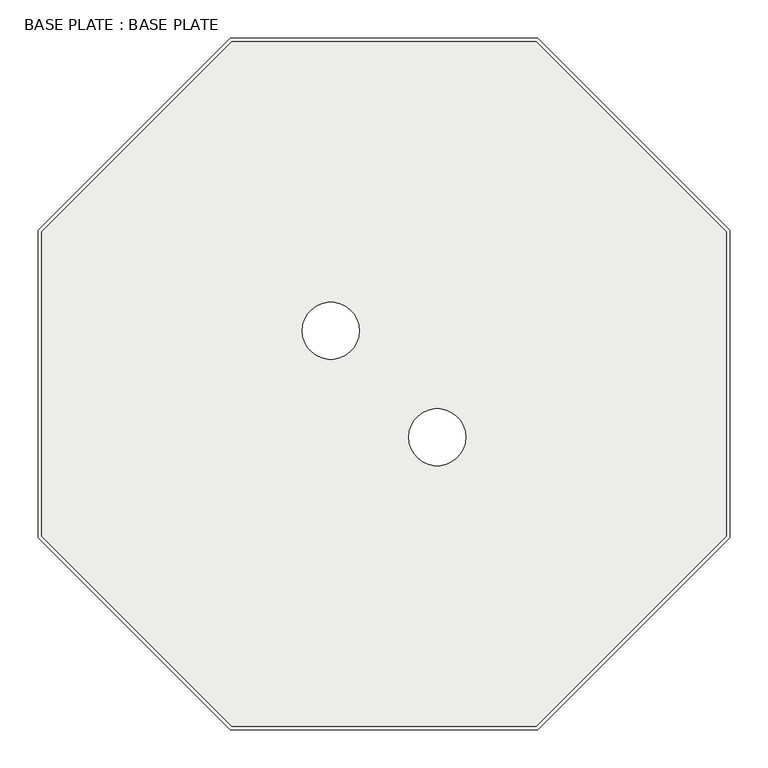
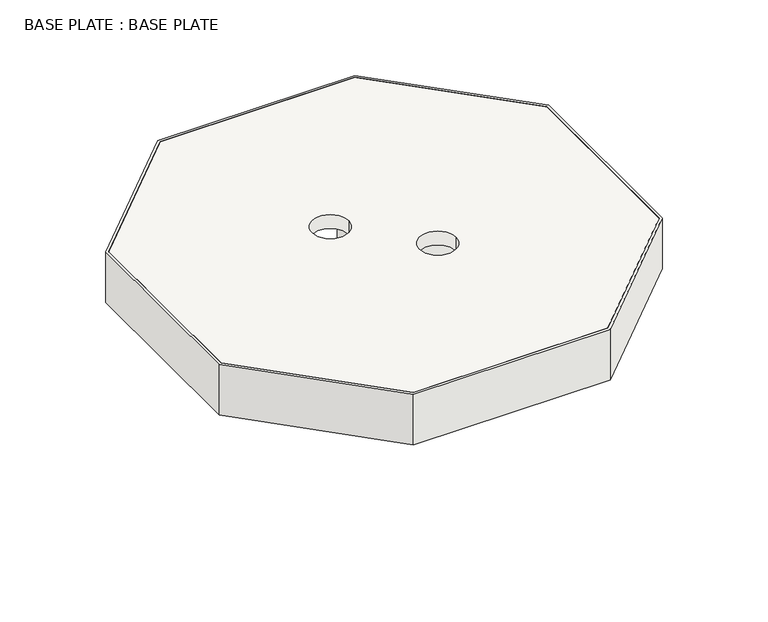
"""IFC4 building model written with IfcOpenShell, lengths in millimetres: slab geometry, BASE PLATE : BASE PLATE."""

from ifc_helpers import new_model, si_unit, point, frame, frame_2d, origin, place, context, project, spatial, polyline, circle_curve, trimmed, segment, composite_curve, outline, extrude, source, transform, mapped, element, save


def base_plate_base_plate_fc0de6f1(model_context):
    return source(origin(), model_context, "Body", "SweptSolid", [
        extrude(outline(polyline([(455.0, 19297.4497911), (202.0710678, 19044.5208589), (-202.0710678, 19044.5208589), (-455.0, 19297.4497911), (-455.0, 19701.5919267), (-202.0710678, 19954.5208589), (202.0710678, 19954.5208589), (455.0, 19701.5919267), (455.0, 19297.4497911)]), holes=[polyline([(-450.0, 19299.5208589), (-200.0, 19049.5208589), (200.0, 19049.5208589), (450.0, 19299.5208589), (450.0, 19699.5208589), (200.0, 19949.5208589), (-200.0, 19949.5208589), (-450.0, 19699.5208589), (-450.0, 19299.5208589)])]), frame((0.0, 0.0, 210.0), z_axis=(0.0, 0.0, 1.0), x_axis=(1.0, 0.0, 0.0)), (0.0, 0.0, 1.0), 110.0),
        extrude(outline(polyline([(-150.0, 19489.5208589), (-150.0, 19499.5208589), (-150.0, 19509.5208589), (-10.0, 19509.5208589), (-10.0, 19649.5208589), (10.0, 19649.5208589), (10.0, 19509.5208589), (150.0, 19509.5208589), (150.0, 19489.5208589), (10.0, 19489.5208589), (10.0, 19349.5208589), (-10.0, 19349.5208589), (-10.0, 19489.5208589), (-150.0, 19489.5208589)])), frame((0.0, 0.0, -10.0), z_axis=(0.0, 0.0, 1.0), x_axis=(1.0, 0.0, 0.0)), (0.0, 0.0, 1.0), 300.0),
        extrude(outline(polyline([(450.0, 19699.5208589), (450.0, 19299.5208589), (200.0, 19049.5208589), (-200.0, 19049.5208589), (-450.0, 19299.5208589), (-450.0, 19699.5208589), (-200.0, 19949.5208589), (200.0, 19949.5208589), (450.0, 19699.5208589)]), holes=[composite_curve([segment(trimmed(circle_curve(frame_2d((70.0, 19429.5208589)), 37.5), [point((32.5, 19429.5208589))], [point((107.5, 19429.5208589))], True, "CARTESIAN"), True, "CONTINUOUS"), segment(trimmed(circle_curve(frame_2d((70.0, 19429.5208589)), 37.5), [point((107.5, 19429.5208589))], [point((32.5, 19429.5208589))], True, "CARTESIAN"), True, "CONTINUOUS")], self_intersect=False), composite_curve([segment(trimmed(circle_curve(frame_2d((-70.0, 19569.5208589)), 37.5), [point((-107.5, 19569.5208589))], [point((-32.5, 19569.5208589))], True, "CARTESIAN"), True, "CONTINUOUS"), segment(trimmed(circle_curve(frame_2d((-70.0, 19569.5208589)), 37.5), [point((-32.5, 19569.5208589))], [point((-107.5, 19569.5208589))], True, "CARTESIAN"), True, "CONTINUOUS")], self_intersect=False)]), frame((0.0, 0.0, 290.0), z_axis=(0.0, 0.0, 1.0), x_axis=(1.0, 0.0, 0.0)), (0.0, 0.0, 1.0), 30.0),
    ])


if __name__ == "__main__":
    model = new_model("IFC4")
    model_context = context("Model", 3, world=origin())
    ifc_project = project(units=[si_unit("LENGTHUNIT", "METRE", prefix="MILLI")], contexts=[model_context])
    site = spatial("IfcSite", under=ifc_project)
    building = spatial("IfcBuilding", under=site)
    placement = place(None, origin())
    base_plate_base_plate_shape = base_plate_base_plate_fc0de6f1(model_context)
    element("IfcSlab", 1, ObjectType="BASE PLATE : BASE PLATE", at=placement, inside=building, context=model_context, shape_type="MappedRepresentation", body=[
        mapped(base_plate_base_plate_shape, transform((0.0, 0.0, 0.0), x_axis=(1.0, 0.0, 0.0), y_axis=(0.0, 1.0, 0.0), z_axis=(0.0, 0.0, 1.0))),
    ])
    save(model, "model.ifc")
